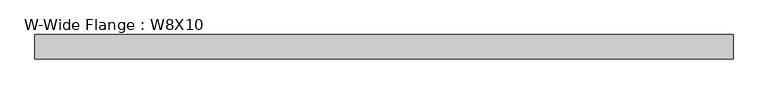
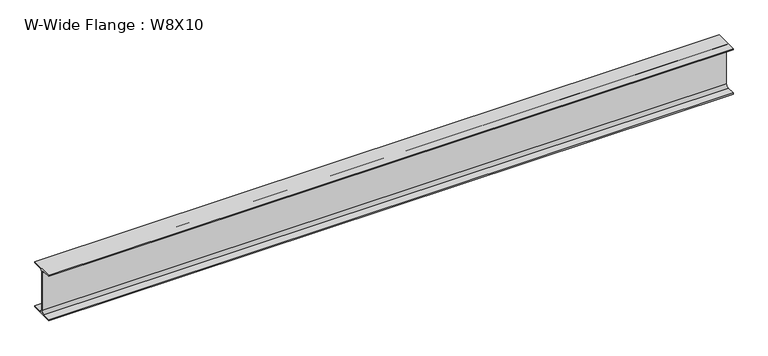
"""IFC4 building model written with IfcOpenShell, lengths in millimetres: beam geometry, W-Wide Flange : W8X10."""

from ifc_helpers import new_model, si_unit, point, frame, frame_2d, origin, place, context, project, spatial, polyline, circle_curve, trimmed, segment, composite_curve, outline, extrude, source, transform, mapped, element, save


def w_wide_flange_w8x10_0a1c7429(model_context):
    return source(origin(), model_context, "Body", "SweptSolid", [
        extrude(outline(composite_curve([segment(polyline([(50.038, -94.996), (50.038, -100.203), (-50.038, -100.203), (-50.038, -94.996), (-14.4145, -94.996)]), True, "CONTINUOUS"), segment(trimmed(circle_curve(frame_2d((-14.4145, -82.7405)), 12.2555), [point((-14.4145, -94.996))], [point((-2.159, -82.7405))], True, "CARTESIAN"), True, "CONTINUOUS"), segment(polyline([(-2.159, -82.7405), (-2.159, 82.7405)]), True, "CONTINUOUS"), segment(trimmed(circle_curve(frame_2d((-14.4145, 82.7405)), 12.2555), [point((-2.159, 82.7405))], [point((-14.4145, 94.996))], True, "CARTESIAN"), True, "CONTINUOUS"), segment(polyline([(-14.4145, 94.996), (-50.038, 94.996), (-50.038, 100.203), (50.038, 100.203), (50.038, 94.996), (14.4145, 94.996)]), True, "CONTINUOUS"), segment(trimmed(circle_curve(frame_2d((14.4145, 82.7405)), 12.2555), [point((14.4145, 94.996))], [point((2.159, 82.7405))], True, "CARTESIAN"), True, "CONTINUOUS"), segment(polyline([(2.159, 82.7405), (2.159, -82.7405)]), True, "CONTINUOUS"), segment(trimmed(circle_curve(frame_2d((14.4145, -82.7405)), 12.2555), [point((2.159, -82.7405))], [point((14.4145, -94.996))], True, "CARTESIAN"), True, "CONTINUOUS"), segment(polyline([(14.4145, -94.996), (50.038, -94.996)]), True, "CONTINUOUS")], self_intersect=False)), frame((-1117.6, 0.0, 0.0), z_axis=(1.0, 0.0, 0.0), x_axis=(0.0, 1.0, 0.0)), (0.0, 0.0, 1.0), 2854.1219816),
    ])


if __name__ == "__main__":
    model = new_model("IFC4")
    model_context = context("Model", 3, world=origin())
    ifc_project = project(units=[si_unit("LENGTHUNIT", "METRE", prefix="MILLI")], contexts=[model_context])
    site = spatial("IfcSite", under=ifc_project)
    building = spatial("IfcBuilding", under=site)
    placement = place(None, origin())
    w_wide_flange_w8x10_shape = w_wide_flange_w8x10_0a1c7429(model_context)
    element("IfcBeam", 1, ObjectType="W-Wide Flange : W8X10", at=placement, inside=building, context=model_context, shape_type="MappedRepresentation", body=[
        mapped(w_wide_flange_w8x10_shape, transform((0.0, 0.0, 0.0), x_axis=(1.0, 0.0, 0.0), y_axis=(0.0, 1.0, 0.0), z_axis=(0.0, 0.0, 1.0))),
    ])
    save(model, "model.ifc")

# Revit data of these elements
# Project information
#   Project Issue Date = "10/18/2018"
#   Project Status = "Project Status"
#   Client Name = "Owner"
#   Project Address = "OPTION - 1 & OPTION 2"
#   Project Name = "ORGANIC GROCERY STORE"
#   Project Number = "Project Number"
# Type "W-Wide Flange : W8X10"
#   Assembly Code = "B10"
#   W = 10
#   Length [instance default] = 5' - 0"
#   bf = 0' - 3.94"
#   d = 0' - 7.89"
#   k = 0' - 0 11/16"
#   k2 = 0' - 0.4825"
#   tf = 0' - 0.205"
#   tw = 0' - 0.17"
#   A = 0.0205556 SF
#   Structural Material [instance default] = Steel ASTM A992
# Element 1 (IfcBeam, "W-Wide Flange : W8X10")
#   Structural Material = none
# Materials
#   "Steel ASTM A992": class "Metal", colour RGB 189 187 185, transparency 0, Description = "Structural steel 50ksi", Cost = 0
